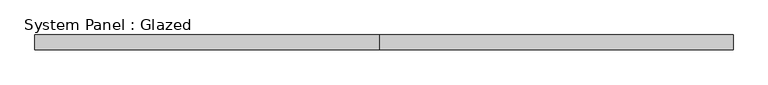
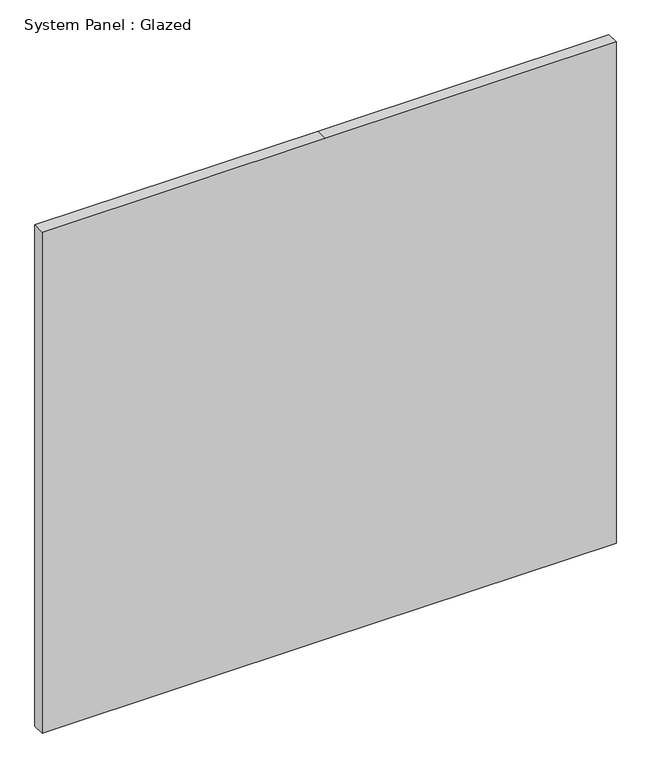
"""IFC4 building model written with IfcOpenShell, lengths in millimetres: plate geometry, System Panel : Glazed."""

import ifcopenshell
import ifcopenshell.guid

model = None  # the IFC model being written
_history = None  # IfcOwnerHistory: only IFC2X3 demands one
_inside = {}  # id of a spatial element -> (the spatial element, [elements in it])
_under = {}  # id of a project, library or spatial element -> (it, [spatial elements below it])
_declared = {}  # id of a project -> (the project, [libraries it declares])
_typed = {}  # id of a type object -> (the type object, [elements of that type])
_made_of = {}  # id of a material, layer set ... -> (it, [elements and type objects made of it])


def new_model(schema):
    """Start an empty IFC model of exactly this schema.

    Asked for "IFC4X3", IfcOpenShell would pick the latest addendum, in which some entities
    have other attributes; the version numbers below select the first issue.
    IFC2X3 requires an IfcOwnerHistory on every rooted entity: one is made here for all.
    """
    global model, _history
    if schema == "IFC4X3":
        model = ifcopenshell.file(schema_version=(4, 3, 0, 0))
    else:
        model = ifcopenshell.file(schema=schema)
    _inside.clear()
    _under.clear()
    _declared.clear()
    _typed.clear()
    _made_of.clear()
    _history = None
    if model.schema == "IFC2X3":
        org = make("IfcOrganization", Name="unknown")
        user = make(
            "IfcPersonAndOrganization",
            ThePerson=make("IfcPerson", FamilyName="unknown"),
            TheOrganization=org,
        )
        app = make(
            "IfcApplication",
            ApplicationDeveloper=org,
            Version="unknown",
            ApplicationFullName="unknown",
            ApplicationIdentifier="unknown",
        )
        _history = make(
            "IfcOwnerHistory",
            OwningUser=user,
            OwningApplication=app,
            ChangeAction="ADDED",
            CreationDate=0,
        )
    return model


def make(cls, **values):
    """One entity of the class cls with the attributes given. An attribute that is None is left unset."""
    return model.create_entity(
        cls, **{name: value for name, value in values.items() if value is not None}
    )


def rooted(cls, **values):
    """An entity with a GlobalId (a new one), such as an element, a storey or a relation."""
    return make(cls, GlobalId=ifcopenshell.guid.new(), OwnerHistory=_history, **values)


def si_unit(unit_type, name, prefix=None):
    """IfcSIUnit, for example si_unit("LENGTHUNIT", "METRE", prefix="MILLI")."""
    return make("IfcSIUnit", UnitType=unit_type, Prefix=prefix, Name=name)


def assignment(units):
    """IfcUnitAssignment: the units of a project."""
    return None if units is None else make("IfcUnitAssignment", Units=units)


def point(xyz):
    """IfcCartesianPoint."""
    return None if xyz is None else make("IfcCartesianPoint", Coordinates=xyz)


def direction(xyz):
    """IfcDirection."""
    return None if xyz is None else make("IfcDirection", DirectionRatios=xyz)


def frame(location, z_axis=None, x_axis=None):
    """IfcAxis2Placement3D, a coordinate frame: its origin and axes. An axis left out is left unset."""
    return make(
        "IfcAxis2Placement3D",
        Location=point(location),
        Axis=direction(z_axis),
        RefDirection=direction(x_axis),
    )


def origin():
    """The frame at (0, 0, 0) with its axes left unset."""
    return frame((0.0, 0.0, 0.0))


def place(relative_to, where):
    """IfcLocalPlacement: puts the frame where relative to a parent placement (None: the world)."""
    return make(
        "IfcLocalPlacement", PlacementRelTo=relative_to, RelativePlacement=where
    )


def context(
    kind, dimensions, precision=None, world=None, true_north=None, identifier=None
):
    """IfcGeometricRepresentationContext, for example the 3D "Model" context."""
    return make(
        "IfcGeometricRepresentationContext",
        ContextIdentifier=identifier,
        ContextType=kind,
        CoordinateSpaceDimension=dimensions,
        Precision=precision,
        WorldCoordinateSystem=world,
        TrueNorth=true_north,
    )


def project(units=None, contexts=None):
    """IfcProject with its units and contexts."""
    return rooted(
        "IfcProject",
        Name="project",
        RepresentationContexts=contexts,
        UnitsInContext=assignment(units),
    )


def spatial(cls, under=None, at=None, **own):
    """A site, building, storey or space (cls), placed at a placement, below another one or the project."""
    s = rooted(cls, ObjectPlacement=at, **own)
    if under is not None:
        _under.setdefault(under.id(), (under, []))[1].append(s)
    return s


def polyline(points):
    """IfcPolyline through the points."""
    return make("IfcPolyline", Points=[point(p) for p in points])


def outline(outer, holes=None, kind="AREA"):
    """IfcArbitraryClosedProfileDef: a profile drawn as a closed curve; with holes, ...WithVoids."""
    if holes is None:
        return make("IfcArbitraryClosedProfileDef", ProfileType=kind, OuterCurve=outer)
    return make(
        "IfcArbitraryProfileDefWithVoids",
        ProfileType=kind,
        OuterCurve=outer,
        InnerCurves=holes,
    )


def extrude(swept, where, along, depth):
    """IfcExtrudedAreaSolid: the profile swept, set in the frame where, extruded along a direction by depth."""
    return make(
        "IfcExtrudedAreaSolid",
        SweptArea=swept,
        Position=where,
        ExtrudedDirection=direction(along),
        Depth=depth,
    )


def shape(context_of_items, identifier, shape_type, items):
    """IfcShapeRepresentation: the items that make up one representation, for example the "Body"."""
    return make(
        "IfcShapeRepresentation",
        ContextOfItems=context_of_items,
        RepresentationIdentifier=identifier,
        RepresentationType=shape_type,
        Items=items,
    )


def source(mapping_origin, context_of_items, identifier, shape_type, items):
    """IfcRepresentationMap: a shape defined once, which mapped items show again and again."""
    return make(
        "IfcRepresentationMap",
        MappingOrigin=mapping_origin,
        MappedRepresentation=shape(context_of_items, identifier, shape_type, items),
    )


def transform(
    local_origin,
    x_axis=None,
    y_axis=None,
    z_axis=None,
    scale=None,
    scale2=None,
    scale3=None,
    uniform=True,
):
    """IfcCartesianTransformationOperator3D, or its non-uniform kind. x_axis, y_axis, z_axis: its Axis1, 2, 3."""
    if uniform:
        return make(
            "IfcCartesianTransformationOperator3D",
            Axis1=direction(x_axis),
            Axis2=direction(y_axis),
            LocalOrigin=point(local_origin),
            Scale=scale,
            Axis3=direction(z_axis),
        )
    return make(
        "IfcCartesianTransformationOperator3DnonUniform",
        Axis1=direction(x_axis),
        Axis2=direction(y_axis),
        LocalOrigin=point(local_origin),
        Scale=scale,
        Axis3=direction(z_axis),
        Scale2=scale2,
        Scale3=scale3,
    )


def mapped(mapping_source, mapping_target):
    """IfcMappedItem: shows the shape of a source again, moved by a transform."""
    return make(
        "IfcMappedItem", MappingSource=mapping_source, MappingTarget=mapping_target
    )


def made_of(thing, what):
    """Note that an element or type object is made of a material, layer set ...; save() writes the relation."""
    if what is not None:
        _made_of.setdefault(what.id(), (what, []))[1].append(thing)
    return thing


def element(
    cls,
    number,
    at=None,
    inside=None,
    cuts=None,
    type_object=None,
    material=None,
    context=None,
    identifier="Body",
    shape_type=None,
    held_by="IfcProductDefinitionShape",
    body=None,
    shapes=None,
    **own,
):
    """One element of the class cls, such as IfcWall. Its Tag is "e" and its number.

    at: its placement. inside: the storey or other place that contains it. cuts: it is an
    opening in that element (IfcRelVoidsElement). A single representation is given by context,
    identifier, shape_type and body (its items); several are given by shapes. held_by: the class
    of the entity that holds the representations. save() writes the other relations.
    """
    e = rooted(cls, Tag="e%d" % number, ObjectPlacement=at, **own)
    if body is not None:
        shapes = [shape(context, identifier, shape_type, body)]
    if shapes is not None:
        e.Representation = make(held_by, Representations=shapes)
    if inside is not None:
        _inside.setdefault(inside.id(), (inside, []))[1].append(e)
    if cuts is not None:
        rooted(
            "IfcRelVoidsElement", RelatingBuildingElement=cuts, RelatedOpeningElement=e
        )
    if type_object is not None:
        _typed.setdefault(type_object.id(), (type_object, []))[1].append(e)
    return made_of(e, material)


def aggregate(whole, parts):
    """IfcRelAggregates: a whole, such as a stair, and the parts it consists of."""
    return rooted("IfcRelAggregates", RelatingObject=whole, RelatedObjects=parts)


def save(model, path):
    """Write the relations noted so far, then the file.

    IfcRelAggregates (storeys below a building ...), IfcRelContainedInSpatialStructure (elements
    in a storey), IfcRelDefinesByType, IfcRelAssociatesMaterial and IfcRelDeclares: one each for
    every whole, place, type object, material and project.
    """
    for whole, parts in _under.values():
        aggregate(whole, parts)
    for where, things in _inside.values():
        rooted(
            "IfcRelContainedInSpatialStructure",
            RelatedElements=things,
            RelatingStructure=where,
        )
    for kind, things in _typed.values():
        rooted("IfcRelDefinesByType", RelatedObjects=things, RelatingType=kind)
    for what, things in _made_of.values():
        rooted("IfcRelAssociatesMaterial", RelatedObjects=things, RelatingMaterial=what)
    for by, libraries in _declared.values():
        rooted("IfcRelDeclares", RelatingContext=by, RelatedDefinitions=libraries)
    model.write(path)


def system_panel_glazed_820f17d5(model_context):
    return source(origin(), model_context, "Body", "SweptSolid", [
        extrude(outline(polyline([(0.0, -1164.932565), (0.0, -14.932565), (0.0, 1164.932565), (2150.0, 1164.932565), (2150.0, -14.932565), (2150.0, -1164.932565), (0.0, -1164.932565)])), frame((0.0, -25.0, 0.0), z_axis=(0.0, 1.0, 0.0), x_axis=(0.0, 0.0, 1.0)), (0.0, 0.0, 1.0), 50.0),
    ])


if __name__ == "__main__":
    model = new_model("IFC4")
    model_context = context("Model", 3, world=origin())
    ifc_project = project(units=[si_unit("LENGTHUNIT", "METRE", prefix="MILLI")], contexts=[model_context])
    site = spatial("IfcSite", under=ifc_project)
    building = spatial("IfcBuilding", under=site)
    placement = place(None, origin())
    system_panel_glazed_shape = system_panel_glazed_820f17d5(model_context)
    element("IfcPlate", 1, ObjectType="System Panel : Glazed", at=placement, inside=building, context=model_context, shape_type="MappedRepresentation", body=[
        mapped(system_panel_glazed_shape, transform((0.0, 0.0, 0.0), x_axis=(1.0, 0.0, 0.0), y_axis=(0.0, 1.0, 0.0), z_axis=(0.0, 0.0, 1.0))),
    ])
    save(model, "model.ifc")

# Revit data of these elements
# Type "System Panel : Glazed"
#   Type Mark = "CW-GLASS"
# Element 1 (IfcPlate, "System Panel : Glazed")
#   Materials on its faces: "Glass_Clear"
# Materials
#   "Glass_Clear": class "Glass", colour RGB 128 128 255, transparency 0.8, Comments = "Rendering appearance not upgraded ", Cost = 0
